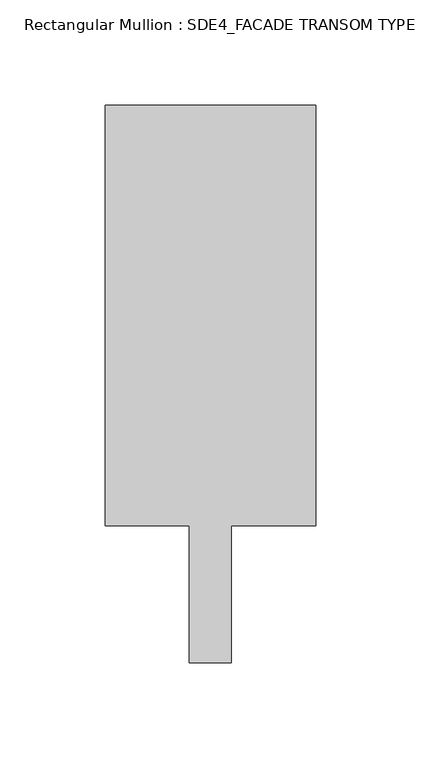
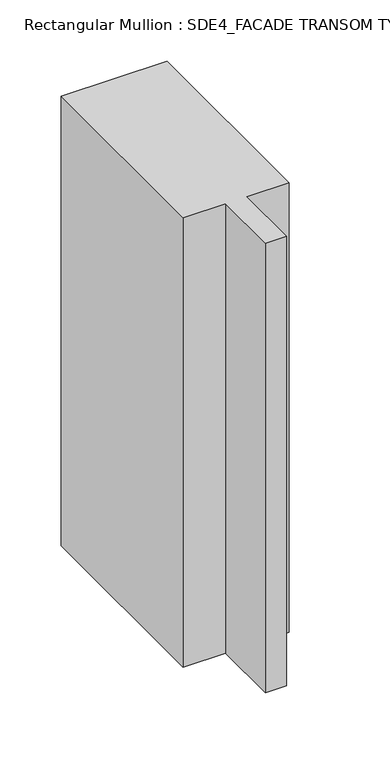
"""IFC4 building model written with IfcOpenShell, lengths in millimetres: member geometry, Rectangular Mullion : SDE4_FACADE TRANSOM TYPE 2."""

from ifc_helpers import new_model, si_unit, frame, origin, place, context, project, spatial, polyline, outline, extrude, source, transform, mapped, element, save


def rectangular_mullion_sde4_facade_transom_type_2_5f4c2513(model_context):
    return source(origin(), model_context, "Body", "SweptSolid", [
        extrude(outline(polyline([(50.0, 132.5), (50.0, -67.5), (10.0, -67.5), (10.0, -132.5), (-10.0, -132.5), (-10.0, -67.5), (-50.0, -67.5), (-50.0, 132.5), (50.0, 132.5)])), frame((0.0, 0.0, -448.9493952), z_axis=(0.0, 0.0, 1.0), x_axis=(1.0, 0.0, 0.0)), (0.0, 0.0, 1.0), 448.9493952),
    ])


if __name__ == "__main__":
    model = new_model("IFC4")
    model_context = context("Model", 3, world=origin())
    ifc_project = project(units=[si_unit("LENGTHUNIT", "METRE", prefix="MILLI")], contexts=[model_context])
    site = spatial("IfcSite", under=ifc_project)
    building = spatial("IfcBuilding", under=site)
    placement = place(None, origin())
    rectangular_mullion_sde4_facade_transom_type_2_shape = rectangular_mullion_sde4_facade_transom_type_2_5f4c2513(model_context)
    element("IfcMember", 1, ObjectType="Rectangular Mullion : SDE4_FACADE TRANSOM TYPE 2", at=placement, inside=building, context=model_context, shape_type="MappedRepresentation", body=[
        mapped(rectangular_mullion_sde4_facade_transom_type_2_shape, transform((0.0, 0.0, 0.0), x_axis=(1.0, 0.0, 0.0), y_axis=(0.0, 1.0, 0.0), z_axis=(0.0, 0.0, 1.0))),
    ])
    save(model, "model.ifc")

# Revit data of these elements
# Type "Rectangular Mullion : SDE4_FACADE TRANSOM TYPE 2"
#   built-in parameter 1007322 = 0.869423 (stored number, unit not read)
#   built-in parameter 1007321 = 0.164042 (stored number, unit not read)
#   built-in parameter 1007320 = 0.164042 (stored number, unit not read)
